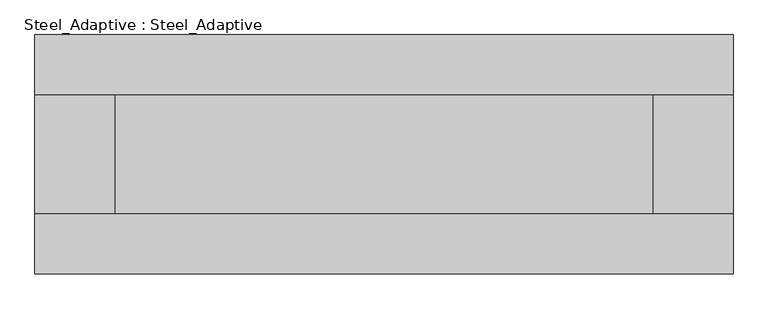
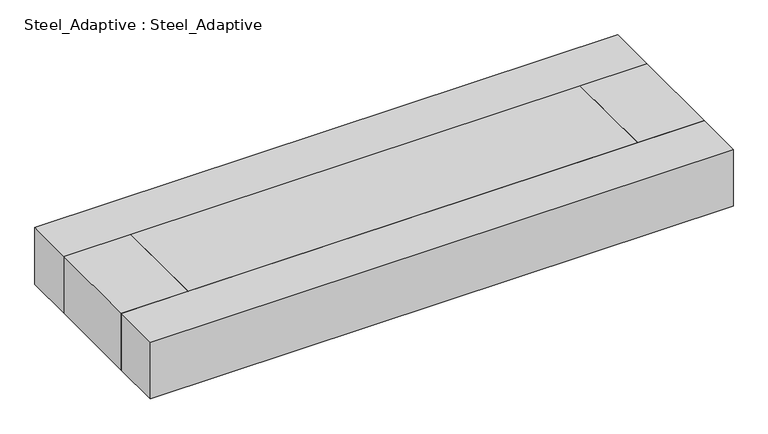
"""IFC4 building model written with IfcOpenShell, lengths in millimetres: proxy geometry, Steel_Adaptive : Steel_Adaptive."""

from ifc_helpers import new_model, si_unit, frame, origin, place, context, project, spatial, polyline, outline, extrude, source, transform, mapped, element, save


def steel_adaptive_steel_adaptive_8ee894f9(model_context):
    return source(origin(), model_context, "Body", "SweptSolid", [
        extrude(outline(polyline([(8750.0, 1500.0), (-8750.0, 1500.0), (-8750.0, 3000.0), (8750.0, 3000.0), (8750.0, 1500.0)])), frame((0.0, 0.0, 13500.0), z_axis=(0.0, 0.0, 1.0), x_axis=(1.0, 0.0, 0.0)), (0.0, 0.0, 1.0), 1800.0),
        extrude(outline(polyline([(-8750.0, -1500.0), (8750.0, -1500.0), (8750.0, -3000.0), (-8750.0, -3000.0), (-8750.0, -1500.0)])), frame((0.0, 0.0, 13500.0), z_axis=(0.0, 0.0, 1.0), x_axis=(1.0, 0.0, 0.0)), (0.0, 0.0, 1.0), 1800.0),
        extrude(outline(polyline([(6750.0, -1500.0), (6750.0, 1500.0), (8750.0, 1500.0), (8750.0, -1500.0), (6750.0, -1500.0)])), frame((0.0, 0.0, 13500.0), z_axis=(0.0, 0.0, 1.0), x_axis=(1.0, 0.0, 0.0)), (0.0, 0.0, 1.0), 1800.0),
        extrude(outline(polyline([(-6750.0, 1500.0), (-6750.0, -1500.0), (-8750.0, -1500.0), (-8750.0, 1500.0), (-6750.0, 1500.0)])), frame((0.0, 0.0, 13500.0), z_axis=(0.0, 0.0, 1.0), x_axis=(1.0, 0.0, 0.0)), (0.0, 0.0, 1.0), 1800.0),
        extrude(outline(polyline([(-6750.0, -1500.0), (-6750.0, 1500.0), (6750.0, 1500.0), (6750.0, -1500.0), (-6750.0, -1500.0)])), frame((0.0, 0.0, 13500.0), z_axis=(0.0, 0.0, 1.0), x_axis=(1.0, 0.0, 0.0)), (0.0, 0.0, 1.0), 1800.0),
    ])


if __name__ == "__main__":
    model = new_model("IFC4")
    model_context = context("Model", 3, world=origin())
    ifc_project = project(units=[si_unit("LENGTHUNIT", "METRE", prefix="MILLI")], contexts=[model_context])
    site = spatial("IfcSite", under=ifc_project)
    building = spatial("IfcBuilding", under=site)
    placement = place(None, origin())
    steel_adaptive_steel_adaptive_shape = steel_adaptive_steel_adaptive_8ee894f9(model_context)
    element("IfcBuildingElementProxy", 1, Name="Steel_Adaptive : Steel_Adaptive", ObjectType="Steel_Adaptive : Steel_Adaptive", at=placement, inside=building, context=model_context, shape_type="MappedRepresentation", body=[
        mapped(steel_adaptive_steel_adaptive_shape, transform((0.0, 0.0, 0.0), x_axis=(1.0, 0.0, 0.0), y_axis=(0.0, 1.0, 0.0), z_axis=(0.0, 0.0, 1.0))),
    ])
    save(model, "model.ifc")

# Revit data of these elements
# Type "Steel_Adaptive : Steel_Adaptive"
#   Width = 3000 mm
#   Top Width = 3000 mm
#   Length = 21000 mm
#   Height [instance default] = 80000 mm
#   Default Elevation = 0
# Element 1 (IfcBuildingElementProxy, "Steel_Adaptive : Steel_Adaptive")
#   Height = 13500 mm
